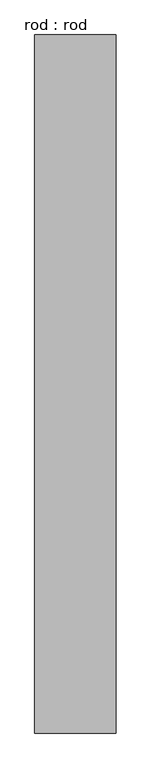
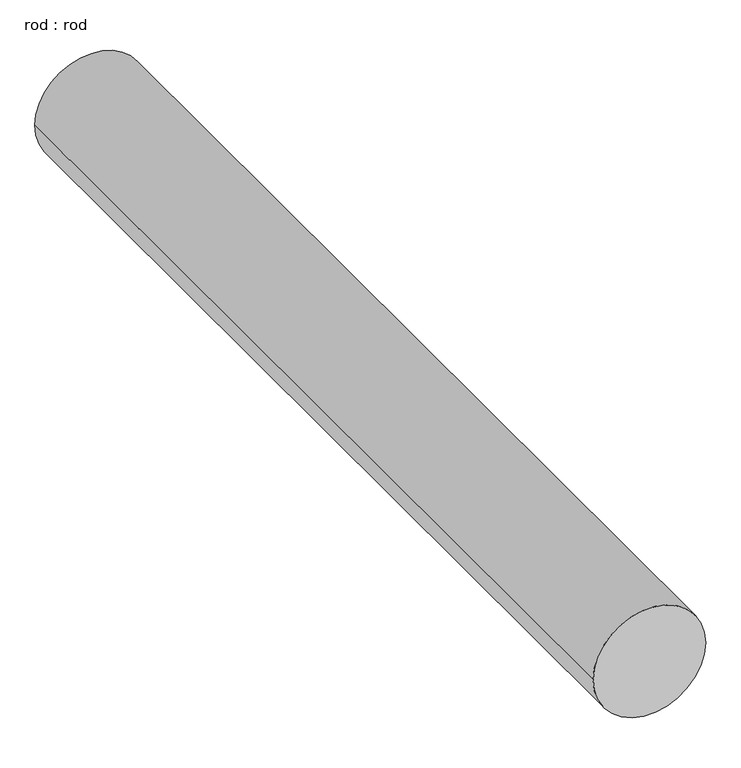
"""IFC4 building model written with IfcOpenShell, lengths in millimetres: proxy geometry, rod : rod."""

from ifc_helpers import new_model, si_unit, point, frame, frame_2d, origin, place, context, project, spatial, circle_curve, trimmed, segment, composite_curve, outline, extrude, source, transform, mapped, element, save


def rod_rod_21cfa642(model_context):
    return source(origin(), model_context, "Body", "SweptSolid", [
        extrude(outline(composite_curve([segment(trimmed(circle_curve(frame_2d((0.0108462, 0.0)), 200.0), [point((0.0108462, 200.0))], [point((0.0108462, -200.0))], False, "CARTESIAN"), True, "CONTINUOUS"), segment(trimmed(circle_curve(frame_2d((0.0108462, 0.0)), 200.0), [point((0.0108462, -200.0))], [point((0.0108462, 200.0))], False, "CARTESIAN"), True, "CONTINUOUS")], self_intersect=False)), frame((0.0, 2372.7286153, 0.0), z_axis=(0.0, 1.0, 0.0), x_axis=(0.0, 0.0, 1.0)), (0.0, 0.0, 1.0), 3440.0),
    ])


if __name__ == "__main__":
    model = new_model("IFC4")
    model_context = context("Model", 3, world=origin())
    ifc_project = project(units=[si_unit("LENGTHUNIT", "METRE", prefix="MILLI")], contexts=[model_context])
    site = spatial("IfcSite", under=ifc_project)
    building = spatial("IfcBuilding", under=site)
    placement = place(None, origin())
    rod_rod_shape = rod_rod_21cfa642(model_context)
    element("IfcBuildingElementProxy", 1, Name="rod : rod", ObjectType="rod : rod", at=placement, inside=building, context=model_context, shape_type="MappedRepresentation", body=[
        mapped(rod_rod_shape, transform((0.0, 0.0, 0.0), x_axis=(1.0, 0.0, 0.0), y_axis=(0.0, 1.0, 0.0), z_axis=(0.0, 0.0, 1.0))),
    ])
    save(model, "model.ifc")

# Revit data of these elements
# Type "rod : rod"
#   Default Elevation = 0
